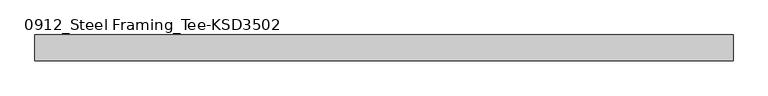
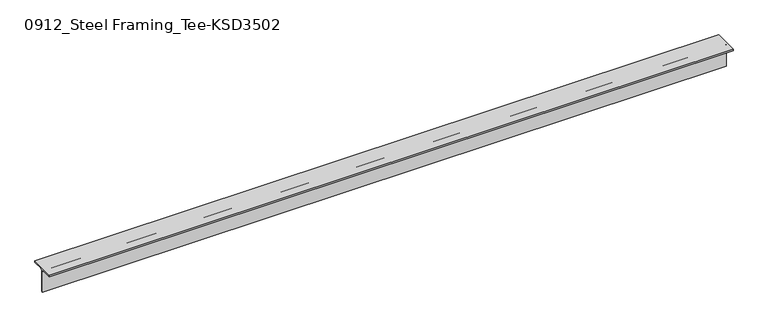
"""IFC4 building model written with IfcOpenShell, lengths in millimetres: member geometry, 0912_Steel Framing_Tee-KSD3502 : H_SB_ASB_CT-150x150x6.5x9."""

import ifcopenshell
import ifcopenshell.guid

model = None  # the IFC model being written
_history = None  # IfcOwnerHistory: only IFC2X3 demands one
_inside = {}  # id of a spatial element -> (the spatial element, [elements in it])
_under = {}  # id of a project, library or spatial element -> (it, [spatial elements below it])
_declared = {}  # id of a project -> (the project, [libraries it declares])
_typed = {}  # id of a type object -> (the type object, [elements of that type])
_made_of = {}  # id of a material, layer set ... -> (it, [elements and type objects made of it])


def new_model(schema):
    """Start an empty IFC model of exactly this schema.

    Asked for "IFC4X3", IfcOpenShell would pick the latest addendum, in which some entities
    have other attributes; the version numbers below select the first issue.
    IFC2X3 requires an IfcOwnerHistory on every rooted entity: one is made here for all.
    """
    global model, _history
    if schema == "IFC4X3":
        model = ifcopenshell.file(schema_version=(4, 3, 0, 0))
    else:
        model = ifcopenshell.file(schema=schema)
    _inside.clear()
    _under.clear()
    _declared.clear()
    _typed.clear()
    _made_of.clear()
    _history = None
    if model.schema == "IFC2X3":
        org = make("IfcOrganization", Name="unknown")
        user = make(
            "IfcPersonAndOrganization",
            ThePerson=make("IfcPerson", FamilyName="unknown"),
            TheOrganization=org,
        )
        app = make(
            "IfcApplication",
            ApplicationDeveloper=org,
            Version="unknown",
            ApplicationFullName="unknown",
            ApplicationIdentifier="unknown",
        )
        _history = make(
            "IfcOwnerHistory",
            OwningUser=user,
            OwningApplication=app,
            ChangeAction="ADDED",
            CreationDate=0,
        )
    return model


def make(cls, **values):
    """One entity of the class cls with the attributes given. An attribute that is None is left unset."""
    return model.create_entity(
        cls, **{name: value for name, value in values.items() if value is not None}
    )


def rooted(cls, **values):
    """An entity with a GlobalId (a new one), such as an element, a storey or a relation."""
    return make(cls, GlobalId=ifcopenshell.guid.new(), OwnerHistory=_history, **values)


def si_unit(unit_type, name, prefix=None):
    """IfcSIUnit, for example si_unit("LENGTHUNIT", "METRE", prefix="MILLI")."""
    return make("IfcSIUnit", UnitType=unit_type, Prefix=prefix, Name=name)


def assignment(units):
    """IfcUnitAssignment: the units of a project."""
    return None if units is None else make("IfcUnitAssignment", Units=units)


def point(xyz):
    """IfcCartesianPoint."""
    return None if xyz is None else make("IfcCartesianPoint", Coordinates=xyz)


def direction(xyz):
    """IfcDirection."""
    return None if xyz is None else make("IfcDirection", DirectionRatios=xyz)


def frame(location, z_axis=None, x_axis=None):
    """IfcAxis2Placement3D, a coordinate frame: its origin and axes. An axis left out is left unset."""
    return make(
        "IfcAxis2Placement3D",
        Location=point(location),
        Axis=direction(z_axis),
        RefDirection=direction(x_axis),
    )


def frame_2d(location, x_axis=None):
    """IfcAxis2Placement2D, a coordinate frame in the plane: its origin and x axis."""
    return make(
        "IfcAxis2Placement2D", Location=point(location), RefDirection=direction(x_axis)
    )


def origin():
    """The frame at (0, 0, 0) with its axes left unset."""
    return frame((0.0, 0.0, 0.0))


def place(relative_to, where):
    """IfcLocalPlacement: puts the frame where relative to a parent placement (None: the world)."""
    return make(
        "IfcLocalPlacement", PlacementRelTo=relative_to, RelativePlacement=where
    )


def context(
    kind, dimensions, precision=None, world=None, true_north=None, identifier=None
):
    """IfcGeometricRepresentationContext, for example the 3D "Model" context."""
    return make(
        "IfcGeometricRepresentationContext",
        ContextIdentifier=identifier,
        ContextType=kind,
        CoordinateSpaceDimension=dimensions,
        Precision=precision,
        WorldCoordinateSystem=world,
        TrueNorth=true_north,
    )


def project(units=None, contexts=None):
    """IfcProject with its units and contexts."""
    return rooted(
        "IfcProject",
        Name="project",
        RepresentationContexts=contexts,
        UnitsInContext=assignment(units),
    )


def spatial(cls, under=None, at=None, **own):
    """A site, building, storey or space (cls), placed at a placement, below another one or the project."""
    s = rooted(cls, ObjectPlacement=at, **own)
    if under is not None:
        _under.setdefault(under.id(), (under, []))[1].append(s)
    return s


def polyline(points):
    """IfcPolyline through the points."""
    return make("IfcPolyline", Points=[point(p) for p in points])


def circle_curve(where, radius):
    """IfcCircle in the frame where."""
    return make("IfcCircle", Position=where, Radius=radius)


def trimmed(basis, trim1, trim2, sense, master):
    """IfcTrimmedCurve: the piece of a basis curve between two trims."""
    return make(
        "IfcTrimmedCurve",
        BasisCurve=basis,
        Trim1=trim1,
        Trim2=trim2,
        SenseAgreement=sense,
        MasterRepresentation=master,
    )


def segment(curve, same_sense, transition):
    """IfcCompositeCurveSegment."""
    return make(
        "IfcCompositeCurveSegment",
        Transition=transition,
        SameSense=same_sense,
        ParentCurve=curve,
    )


def composite_curve(segments, self_intersect=None):
    """IfcCompositeCurve: segments joined end to end."""
    return make("IfcCompositeCurve", Segments=segments, SelfIntersect=self_intersect)


def outline(outer, holes=None, kind="AREA"):
    """IfcArbitraryClosedProfileDef: a profile drawn as a closed curve; with holes, ...WithVoids."""
    if holes is None:
        return make("IfcArbitraryClosedProfileDef", ProfileType=kind, OuterCurve=outer)
    return make(
        "IfcArbitraryProfileDefWithVoids",
        ProfileType=kind,
        OuterCurve=outer,
        InnerCurves=holes,
    )


def extrude(swept, where, along, depth):
    """IfcExtrudedAreaSolid: the profile swept, set in the frame where, extruded along a direction by depth."""
    return make(
        "IfcExtrudedAreaSolid",
        SweptArea=swept,
        Position=where,
        ExtrudedDirection=direction(along),
        Depth=depth,
    )


def shape(context_of_items, identifier, shape_type, items):
    """IfcShapeRepresentation: the items that make up one representation, for example the "Body"."""
    return make(
        "IfcShapeRepresentation",
        ContextOfItems=context_of_items,
        RepresentationIdentifier=identifier,
        RepresentationType=shape_type,
        Items=items,
    )


def source(mapping_origin, context_of_items, identifier, shape_type, items):
    """IfcRepresentationMap: a shape defined once, which mapped items show again and again."""
    return make(
        "IfcRepresentationMap",
        MappingOrigin=mapping_origin,
        MappedRepresentation=shape(context_of_items, identifier, shape_type, items),
    )


def transform(
    local_origin,
    x_axis=None,
    y_axis=None,
    z_axis=None,
    scale=None,
    scale2=None,
    scale3=None,
    uniform=True,
):
    """IfcCartesianTransformationOperator3D, or its non-uniform kind. x_axis, y_axis, z_axis: its Axis1, 2, 3."""
    if uniform:
        return make(
            "IfcCartesianTransformationOperator3D",
            Axis1=direction(x_axis),
            Axis2=direction(y_axis),
            LocalOrigin=point(local_origin),
            Scale=scale,
            Axis3=direction(z_axis),
        )
    return make(
        "IfcCartesianTransformationOperator3DnonUniform",
        Axis1=direction(x_axis),
        Axis2=direction(y_axis),
        LocalOrigin=point(local_origin),
        Scale=scale,
        Axis3=direction(z_axis),
        Scale2=scale2,
        Scale3=scale3,
    )


def mapped(mapping_source, mapping_target):
    """IfcMappedItem: shows the shape of a source again, moved by a transform."""
    return make(
        "IfcMappedItem", MappingSource=mapping_source, MappingTarget=mapping_target
    )


def made_of(thing, what):
    """Note that an element or type object is made of a material, layer set ...; save() writes the relation."""
    if what is not None:
        _made_of.setdefault(what.id(), (what, []))[1].append(thing)
    return thing


def element(
    cls,
    number,
    at=None,
    inside=None,
    cuts=None,
    type_object=None,
    material=None,
    context=None,
    identifier="Body",
    shape_type=None,
    held_by="IfcProductDefinitionShape",
    body=None,
    shapes=None,
    **own,
):
    """One element of the class cls, such as IfcWall. Its Tag is "e" and its number.

    at: its placement. inside: the storey or other place that contains it. cuts: it is an
    opening in that element (IfcRelVoidsElement). A single representation is given by context,
    identifier, shape_type and body (its items); several are given by shapes. held_by: the class
    of the entity that holds the representations. save() writes the other relations.
    """
    e = rooted(cls, Tag="e%d" % number, ObjectPlacement=at, **own)
    if body is not None:
        shapes = [shape(context, identifier, shape_type, body)]
    if shapes is not None:
        e.Representation = make(held_by, Representations=shapes)
    if inside is not None:
        _inside.setdefault(inside.id(), (inside, []))[1].append(e)
    if cuts is not None:
        rooted(
            "IfcRelVoidsElement", RelatingBuildingElement=cuts, RelatedOpeningElement=e
        )
    if type_object is not None:
        _typed.setdefault(type_object.id(), (type_object, []))[1].append(e)
    return made_of(e, material)


def aggregate(whole, parts):
    """IfcRelAggregates: a whole, such as a stair, and the parts it consists of."""
    return rooted("IfcRelAggregates", RelatingObject=whole, RelatedObjects=parts)


def save(model, path):
    """Write the relations noted so far, then the file.

    IfcRelAggregates (storeys below a building ...), IfcRelContainedInSpatialStructure (elements
    in a storey), IfcRelDefinesByType, IfcRelAssociatesMaterial and IfcRelDeclares: one each for
    every whole, place, type object, material and project.
    """
    for whole, parts in _under.values():
        aggregate(whole, parts)
    for where, things in _inside.values():
        rooted(
            "IfcRelContainedInSpatialStructure",
            RelatedElements=things,
            RelatingStructure=where,
        )
    for kind, things in _typed.values():
        rooted("IfcRelDefinesByType", RelatedObjects=things, RelatingType=kind)
    for what, things in _made_of.values():
        rooted("IfcRelAssociatesMaterial", RelatedObjects=things, RelatingMaterial=what)
    for by, libraries in _declared.values():
        rooted("IfcRelDeclares", RelatingContext=by, RelatedDefinitions=libraries)
    model.write(path)


def member_0912_steel_framing_tee_ksd3502_04386d8b(model_context):
    return source(origin(), model_context, "Body", "SweptSolid", [
        extrude(outline(composite_curve([segment(polyline([(-75.0, 75.0), (75.0, 75.0), (75.0, 66.0), (16.25, 66.0)]), True, "CONTINUOUS"), segment(trimmed(circle_curve(frame_2d((16.25, 53.0)), 13.0), [point((16.25, 66.0))], [point((3.25, 53.0))], True, "CARTESIAN"), True, "CONTINUOUS"), segment(polyline([(3.25, 53.0), (3.25, -75.0), (-3.25, -75.0), (-3.25, 53.0)]), True, "CONTINUOUS"), segment(trimmed(circle_curve(frame_2d((-16.25, 53.0)), 13.0), [point((-3.25, 53.0))], [point((-16.25, 66.0))], True, "CARTESIAN"), True, "CONTINUOUS"), segment(polyline([(-16.25, 66.0), (-75.0, 66.0), (-75.0, 75.0)]), True, "CONTINUOUS")], self_intersect=False)), frame((-2031.05, 0.0, 0.0), z_axis=(1.0, 0.0, 0.0), x_axis=(0.0, 1.0, 0.0)), (0.0, 0.0, 1.0), 4077.8),
    ])


if __name__ == "__main__":
    model = new_model("IFC4")
    model_context = context("Model", 3, world=origin())
    ifc_project = project(units=[si_unit("LENGTHUNIT", "METRE", prefix="MILLI")], contexts=[model_context])
    site = spatial("IfcSite", under=ifc_project)
    building = spatial("IfcBuilding", under=site)
    placement = place(None, origin())
    member_0912_steel_framing_tee_ksd3502_shape = member_0912_steel_framing_tee_ksd3502_04386d8b(model_context)
    element("IfcMember", 1, ObjectType="0912_Steel Framing_Tee-KSD3502 : H_SB_ASB_CT-150x150x6.5x9", at=placement, inside=building, context=model_context, shape_type="MappedRepresentation", body=[
        mapped(member_0912_steel_framing_tee_ksd3502_shape, transform((0.0, 0.0, 0.0), x_axis=(1.0, 0.0, 0.0), y_axis=(0.0, 1.0, 0.0), z_axis=(0.0, 0.0, 1.0))),
    ])
    save(model, "model.ifc")

# Revit data of these elements
# Type "0912_Steel Framing_Tee-KSD3502 : H_SB_ASB_CT-150x150x6.5x9"
#   H_WM Code_1 = "S01AA003-00001 | Main Steel Structure Fabrication Work | Shelter/Building | Light Steel - Standard (30KG/M>Weight) | Material: (   )"
#   H_WM Code_2 = "S03AA029-00001 | Main Steel Structure Erection Work | Shelter/Building | Light Steel (30KG/M>Weight) | Material: (   )"
#   H_WM Code_3 = "S01AA010-00001 | Main Steel Structure Fabrication Work | Shelter/Building | Steel Painting/Coating | for Non-Fireproofed Steel Surface, Surface Preparation, Primer, Second & Final Coat | Material: (   )"
#   H_Q'ty Cal Type Tag = "SB-Q2"
#   Width = 15.0 cm
#   Web Thickness = 0.65 cm
#   Web Fillet = 1.3 cm
#   Section Area = 23.39 cm²
#   Perimeter = 0.60 m²/m
#   Nominal Weight = 18.40 kgf/m
#   Height = 15.0 cm
#   Flange Thickness = 0.9 cm
#   Centroid Vertical = 7.5 cm
#   Centroid Horizontal = 7.5 cm
#   Length [instance default] = 1.5000 m
#   Structural Material [instance default] = Steel, 45-345
#   Warping Constant = (empty or 0)
#   Torsional Moment of Inertia = 0
#   Section Name Key = ""
#   Plastic Modulus weak axis = 0
#   Plastic Modulus strong axis = 0
#   Moment of Inertia weak axis = 0
#   Moment of Inertia strong axis = 0
#   Elastic Modulus weak axis = 0
#   Elastic Modulus strong axis = 0
#   Bolt Spacing = 0
#   Assembly Code = ""
# Element 1 (IfcMember, "0912_Steel Framing_Tee-KSD3502 : H_SB_ASB_CT-150x150x6.5x9")
#   Structural Material = none
# Materials
#   "Steel, 45-345": class "Metal", colour RGB 189 187 185, transparency 0, Description = "Steel 345 MPa", Cost = 0
